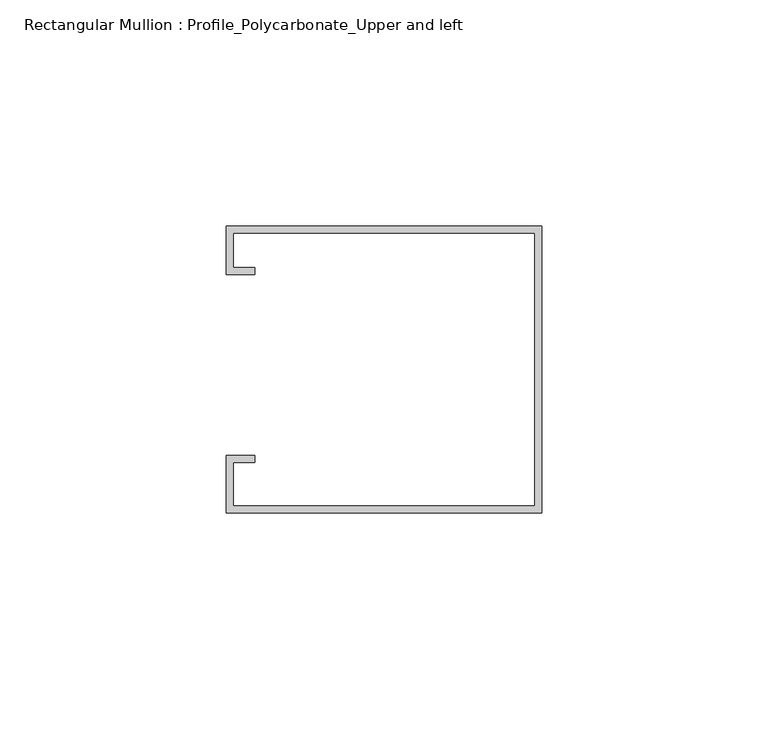
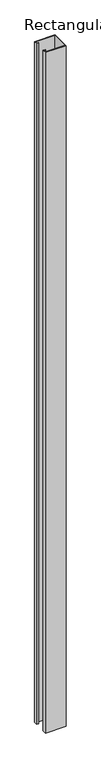
"""IFC4 building model written with IfcOpenShell, lengths in millimetres: member geometry, Rectangular Mullion : Profile_Polycarbonate_Upper and left."""

from ifc_helpers import new_model, si_unit, frame, origin, place, context, project, spatial, polyline, outline, extrude, source, transform, mapped, element, save


def rectangular_mullion_profile_polycarbonate_upper_and_left_860d514b(model_context):
    return source(origin(), model_context, "Body", "SweptSolid", [
        extrude(outline(polyline([(0.0, -32.7), (-69.85, -32.7), (-69.85, -20.0), (-63.5, -20.0), (-63.5, -21.5875), (-68.2625, -21.5875), (-68.2625, -31.1125), (-1.5875, -31.1125), (-1.5875, 29.2125), (-68.2625, 29.2125), (-68.2625, 21.5875), (-63.5, 21.5875), (-63.5, 20.0), (-69.85, 20.0), (-69.85, 30.8), (0.0, 30.8), (0.0, -32.7)])), frame((0.0, 0.0, -2457.6492241), z_axis=(0.0, 0.0, 1.0), x_axis=(1.0, 0.0, 0.0)), (0.0, 0.0, 1.0), 2457.6492241),
    ])


if __name__ == "__main__":
    model = new_model("IFC4")
    model_context = context("Model", 3, world=origin())
    ifc_project = project(units=[si_unit("LENGTHUNIT", "METRE", prefix="MILLI")], contexts=[model_context])
    site = spatial("IfcSite", under=ifc_project)
    building = spatial("IfcBuilding", under=site)
    placement = place(None, origin())
    rectangular_mullion_profile_polycarbonate_upper_and_left_shape = rectangular_mullion_profile_polycarbonate_upper_and_left_860d514b(model_context)
    element("IfcMember", 1, ObjectType="Rectangular Mullion : Profile_Polycarbonate_Upper and left", at=placement, inside=building, context=model_context, shape_type="MappedRepresentation", body=[
        mapped(rectangular_mullion_profile_polycarbonate_upper_and_left_shape, transform((0.0, 0.0, 0.0), x_axis=(1.0, 0.0, 0.0), y_axis=(0.0, 1.0, 0.0), z_axis=(0.0, 0.0, 1.0))),
    ])
    save(model, "model.ifc")

# Revit data of these elements
# Type "Rectangular Mullion : Profile_Polycarbonate_Upper and left"
#   built-in parameter 1007322 = 0.208333 (stored number, unit not read)
#   built-in parameter 1007321 = 0.00520833 (stored number, unit not read)
#   built-in parameter 1007320 = 0 (stored number, unit not read)
# Element 1 (IfcMember, "Rectangular Mullion : Profile_Polycarbonate_Upper and left")
#   Materials on its faces: "ALUMINUM PROFILE AT POLYCARBONATE PANEL"
# Materials
#   "ALUMINUM PROFILE AT POLYCARBONATE PANEL": class "Metal", colour RGB 244 244 244, transparency 0, Description = "Aluminum 6061", Cost = 0
